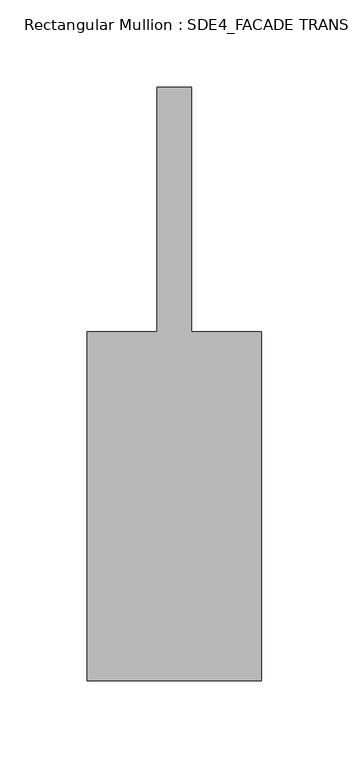
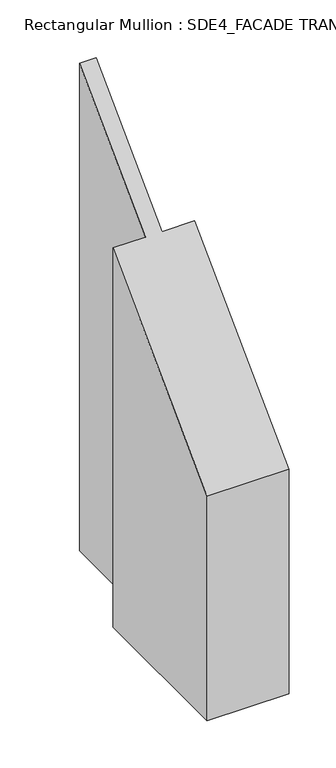
"""IFC4 building model written with IfcOpenShell, lengths in millimetres: member geometry, Rectangular Mullion : SDE4_FACADE TRANSOM TYPE 1."""

from ifc_helpers import new_model, si_unit, origin, place, context, project, spatial, faceted_brep, source, transform, mapped, element, save


def rectangular_mullion_sde4_facade_transom_type_1_ca405e27(model_context):
    return source(origin(), model_context, "Body", "Brep", [
        faceted_brep([(50.0, -132.5, -423.2805066), (-50.0, -132.5, -423.2805066), (-50.0, 67.5, -423.2805066), (-10.0, 67.5, -423.2805066), (-10.0, 207.5, -423.2805066), (10.0, 207.5, -423.2805066), (10.0, 67.5, -423.2805066), (50.0, 67.5, -423.2805066), (50.0, 67.5, 67.5), (50.0, -132.5, -132.5), (10.0, 67.5, 67.5), (10.0, 207.5, 207.5), (-10.0, 207.5, 207.5), (-10.0, 67.5, 67.5), (-50.0, 67.5, 67.5), (-50.0, -132.5, -132.5)], [[[0, 1, 2, 3, 4, 5, 6, 7]], [[8, 9, 0, 7]], [[10, 8, 7, 6]], [[11, 10, 6, 5]], [[12, 11, 5, 4]], [[13, 12, 4, 3]], [[14, 13, 3, 2]], [[15, 14, 2, 1]], [[9, 15, 1, 0]], [[9, 8, 10, 11, 12, 13, 14, 15]]]),
    ])


if __name__ == "__main__":
    model = new_model("IFC4")
    model_context = context("Model", 3, world=origin())
    ifc_project = project(units=[si_unit("LENGTHUNIT", "METRE", prefix="MILLI")], contexts=[model_context])
    site = spatial("IfcSite", under=ifc_project)
    building = spatial("IfcBuilding", under=site)
    placement = place(None, origin())
    rectangular_mullion_sde4_facade_transom_type_1_shape = rectangular_mullion_sde4_facade_transom_type_1_ca405e27(model_context)
    element("IfcMember", 1, ObjectType="Rectangular Mullion : SDE4_FACADE TRANSOM TYPE 1", at=placement, inside=building, context=model_context, shape_type="MappedRepresentation", body=[
        mapped(rectangular_mullion_sde4_facade_transom_type_1_shape, transform((0.0, 0.0, 0.0), x_axis=(1.0, 0.0, 0.0), y_axis=(0.0, 1.0, 0.0), z_axis=(0.0, 0.0, 1.0))),
    ])
    save(model, "model.ifc")

# Revit data of these elements
# Type "Rectangular Mullion : SDE4_FACADE TRANSOM TYPE 1"
#   built-in parameter 1007322 = 1.11549 (stored number, unit not read)
#   built-in parameter 1007321 = 0.164042 (stored number, unit not read)
#   built-in parameter 1007320 = 0.164042 (stored number, unit not read)
